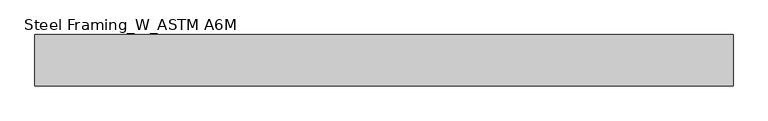
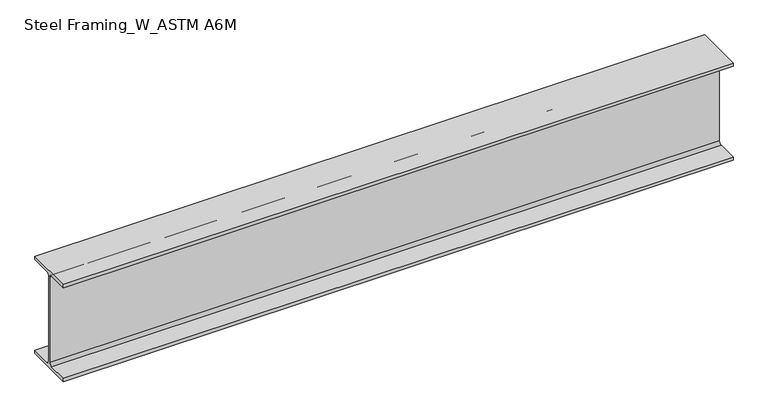
"""IFC4 building model written with IfcOpenShell, lengths in millimetres: beam geometry, Steel Framing_W_ASTM A6M : H_SB_AR_S02_W360x51_G3."""

import ifcopenshell
import ifcopenshell.guid

model = None  # the IFC model being written
_history = None  # IfcOwnerHistory: only IFC2X3 demands one
_inside = {}  # id of a spatial element -> (the spatial element, [elements in it])
_under = {}  # id of a project, library or spatial element -> (it, [spatial elements below it])
_declared = {}  # id of a project -> (the project, [libraries it declares])
_typed = {}  # id of a type object -> (the type object, [elements of that type])
_made_of = {}  # id of a material, layer set ... -> (it, [elements and type objects made of it])


def new_model(schema):
    """Start an empty IFC model of exactly this schema.

    Asked for "IFC4X3", IfcOpenShell would pick the latest addendum, in which some entities
    have other attributes; the version numbers below select the first issue.
    IFC2X3 requires an IfcOwnerHistory on every rooted entity: one is made here for all.
    """
    global model, _history
    if schema == "IFC4X3":
        model = ifcopenshell.file(schema_version=(4, 3, 0, 0))
    else:
        model = ifcopenshell.file(schema=schema)
    _inside.clear()
    _under.clear()
    _declared.clear()
    _typed.clear()
    _made_of.clear()
    _history = None
    if model.schema == "IFC2X3":
        org = make("IfcOrganization", Name="unknown")
        user = make(
            "IfcPersonAndOrganization",
            ThePerson=make("IfcPerson", FamilyName="unknown"),
            TheOrganization=org,
        )
        app = make(
            "IfcApplication",
            ApplicationDeveloper=org,
            Version="unknown",
            ApplicationFullName="unknown",
            ApplicationIdentifier="unknown",
        )
        _history = make(
            "IfcOwnerHistory",
            OwningUser=user,
            OwningApplication=app,
            ChangeAction="ADDED",
            CreationDate=0,
        )
    return model


def make(cls, **values):
    """One entity of the class cls with the attributes given. An attribute that is None is left unset."""
    return model.create_entity(
        cls, **{name: value for name, value in values.items() if value is not None}
    )


def rooted(cls, **values):
    """An entity with a GlobalId (a new one), such as an element, a storey or a relation."""
    return make(cls, GlobalId=ifcopenshell.guid.new(), OwnerHistory=_history, **values)


def si_unit(unit_type, name, prefix=None):
    """IfcSIUnit, for example si_unit("LENGTHUNIT", "METRE", prefix="MILLI")."""
    return make("IfcSIUnit", UnitType=unit_type, Prefix=prefix, Name=name)


def assignment(units):
    """IfcUnitAssignment: the units of a project."""
    return None if units is None else make("IfcUnitAssignment", Units=units)


def point(xyz):
    """IfcCartesianPoint."""
    return None if xyz is None else make("IfcCartesianPoint", Coordinates=xyz)


def direction(xyz):
    """IfcDirection."""
    return None if xyz is None else make("IfcDirection", DirectionRatios=xyz)


def frame(location, z_axis=None, x_axis=None):
    """IfcAxis2Placement3D, a coordinate frame: its origin and axes. An axis left out is left unset."""
    return make(
        "IfcAxis2Placement3D",
        Location=point(location),
        Axis=direction(z_axis),
        RefDirection=direction(x_axis),
    )


def frame_2d(location, x_axis=None):
    """IfcAxis2Placement2D, a coordinate frame in the plane: its origin and x axis."""
    return make(
        "IfcAxis2Placement2D", Location=point(location), RefDirection=direction(x_axis)
    )


def origin():
    """The frame at (0, 0, 0) with its axes left unset."""
    return frame((0.0, 0.0, 0.0))


def place(relative_to, where):
    """IfcLocalPlacement: puts the frame where relative to a parent placement (None: the world)."""
    return make(
        "IfcLocalPlacement", PlacementRelTo=relative_to, RelativePlacement=where
    )


def context(
    kind, dimensions, precision=None, world=None, true_north=None, identifier=None
):
    """IfcGeometricRepresentationContext, for example the 3D "Model" context."""
    return make(
        "IfcGeometricRepresentationContext",
        ContextIdentifier=identifier,
        ContextType=kind,
        CoordinateSpaceDimension=dimensions,
        Precision=precision,
        WorldCoordinateSystem=world,
        TrueNorth=true_north,
    )


def project(units=None, contexts=None):
    """IfcProject with its units and contexts."""
    return rooted(
        "IfcProject",
        Name="project",
        RepresentationContexts=contexts,
        UnitsInContext=assignment(units),
    )


def spatial(cls, under=None, at=None, **own):
    """A site, building, storey or space (cls), placed at a placement, below another one or the project."""
    s = rooted(cls, ObjectPlacement=at, **own)
    if under is not None:
        _under.setdefault(under.id(), (under, []))[1].append(s)
    return s


def polyline(points):
    """IfcPolyline through the points."""
    return make("IfcPolyline", Points=[point(p) for p in points])


def circle_curve(where, radius):
    """IfcCircle in the frame where."""
    return make("IfcCircle", Position=where, Radius=radius)


def trimmed(basis, trim1, trim2, sense, master):
    """IfcTrimmedCurve: the piece of a basis curve between two trims."""
    return make(
        "IfcTrimmedCurve",
        BasisCurve=basis,
        Trim1=trim1,
        Trim2=trim2,
        SenseAgreement=sense,
        MasterRepresentation=master,
    )


def segment(curve, same_sense, transition):
    """IfcCompositeCurveSegment."""
    return make(
        "IfcCompositeCurveSegment",
        Transition=transition,
        SameSense=same_sense,
        ParentCurve=curve,
    )


def composite_curve(segments, self_intersect=None):
    """IfcCompositeCurve: segments joined end to end."""
    return make("IfcCompositeCurve", Segments=segments, SelfIntersect=self_intersect)


def outline(outer, holes=None, kind="AREA"):
    """IfcArbitraryClosedProfileDef: a profile drawn as a closed curve; with holes, ...WithVoids."""
    if holes is None:
        return make("IfcArbitraryClosedProfileDef", ProfileType=kind, OuterCurve=outer)
    return make(
        "IfcArbitraryProfileDefWithVoids",
        ProfileType=kind,
        OuterCurve=outer,
        InnerCurves=holes,
    )


def extrude(swept, where, along, depth):
    """IfcExtrudedAreaSolid: the profile swept, set in the frame where, extruded along a direction by depth."""
    return make(
        "IfcExtrudedAreaSolid",
        SweptArea=swept,
        Position=where,
        ExtrudedDirection=direction(along),
        Depth=depth,
    )


def shape(context_of_items, identifier, shape_type, items):
    """IfcShapeRepresentation: the items that make up one representation, for example the "Body"."""
    return make(
        "IfcShapeRepresentation",
        ContextOfItems=context_of_items,
        RepresentationIdentifier=identifier,
        RepresentationType=shape_type,
        Items=items,
    )


def source(mapping_origin, context_of_items, identifier, shape_type, items):
    """IfcRepresentationMap: a shape defined once, which mapped items show again and again."""
    return make(
        "IfcRepresentationMap",
        MappingOrigin=mapping_origin,
        MappedRepresentation=shape(context_of_items, identifier, shape_type, items),
    )


def transform(
    local_origin,
    x_axis=None,
    y_axis=None,
    z_axis=None,
    scale=None,
    scale2=None,
    scale3=None,
    uniform=True,
):
    """IfcCartesianTransformationOperator3D, or its non-uniform kind. x_axis, y_axis, z_axis: its Axis1, 2, 3."""
    if uniform:
        return make(
            "IfcCartesianTransformationOperator3D",
            Axis1=direction(x_axis),
            Axis2=direction(y_axis),
            LocalOrigin=point(local_origin),
            Scale=scale,
            Axis3=direction(z_axis),
        )
    return make(
        "IfcCartesianTransformationOperator3DnonUniform",
        Axis1=direction(x_axis),
        Axis2=direction(y_axis),
        LocalOrigin=point(local_origin),
        Scale=scale,
        Axis3=direction(z_axis),
        Scale2=scale2,
        Scale3=scale3,
    )


def mapped(mapping_source, mapping_target):
    """IfcMappedItem: shows the shape of a source again, moved by a transform."""
    return make(
        "IfcMappedItem", MappingSource=mapping_source, MappingTarget=mapping_target
    )


def made_of(thing, what):
    """Note that an element or type object is made of a material, layer set ...; save() writes the relation."""
    if what is not None:
        _made_of.setdefault(what.id(), (what, []))[1].append(thing)
    return thing


def element(
    cls,
    number,
    at=None,
    inside=None,
    cuts=None,
    type_object=None,
    material=None,
    context=None,
    identifier="Body",
    shape_type=None,
    held_by="IfcProductDefinitionShape",
    body=None,
    shapes=None,
    **own,
):
    """One element of the class cls, such as IfcWall. Its Tag is "e" and its number.

    at: its placement. inside: the storey or other place that contains it. cuts: it is an
    opening in that element (IfcRelVoidsElement). A single representation is given by context,
    identifier, shape_type and body (its items); several are given by shapes. held_by: the class
    of the entity that holds the representations. save() writes the other relations.
    """
    e = rooted(cls, Tag="e%d" % number, ObjectPlacement=at, **own)
    if body is not None:
        shapes = [shape(context, identifier, shape_type, body)]
    if shapes is not None:
        e.Representation = make(held_by, Representations=shapes)
    if inside is not None:
        _inside.setdefault(inside.id(), (inside, []))[1].append(e)
    if cuts is not None:
        rooted(
            "IfcRelVoidsElement", RelatingBuildingElement=cuts, RelatedOpeningElement=e
        )
    if type_object is not None:
        _typed.setdefault(type_object.id(), (type_object, []))[1].append(e)
    return made_of(e, material)


def aggregate(whole, parts):
    """IfcRelAggregates: a whole, such as a stair, and the parts it consists of."""
    return rooted("IfcRelAggregates", RelatingObject=whole, RelatedObjects=parts)


def save(model, path):
    """Write the relations noted so far, then the file.

    IfcRelAggregates (storeys below a building ...), IfcRelContainedInSpatialStructure (elements
    in a storey), IfcRelDefinesByType, IfcRelAssociatesMaterial and IfcRelDeclares: one each for
    every whole, place, type object, material and project.
    """
    for whole, parts in _under.values():
        aggregate(whole, parts)
    for where, things in _inside.values():
        rooted(
            "IfcRelContainedInSpatialStructure",
            RelatedElements=things,
            RelatingStructure=where,
        )
    for kind, things in _typed.values():
        rooted("IfcRelDefinesByType", RelatedObjects=things, RelatingType=kind)
    for what, things in _made_of.values():
        rooted("IfcRelAssociatesMaterial", RelatedObjects=things, RelatingMaterial=what)
    for by, libraries in _declared.values():
        rooted("IfcRelDeclares", RelatingContext=by, RelatedDefinitions=libraries)
    model.write(path)


def steel_framing_w_astm_a6m_44bd27a9(model_context):
    return source(origin(), model_context, "Body", "SweptSolid", [
        extrude(outline(composite_curve([segment(polyline([(85.5, -166.4), (85.5, -178.0), (-85.5, -178.0), (-85.5, -166.4), (-13.72, -166.4)]), True, "CONTINUOUS"), segment(trimmed(circle_curve(frame_2d((-13.72, -156.3)), 10.1), [point((-13.72, -166.4))], [point((-3.62, -156.3))], True, "CARTESIAN"), True, "CONTINUOUS"), segment(polyline([(-3.62, -156.3), (-3.62, 156.3)]), True, "CONTINUOUS"), segment(trimmed(circle_curve(frame_2d((-13.72, 156.3)), 10.1), [point((-3.62, 156.3))], [point((-13.72, 166.4))], True, "CARTESIAN"), True, "CONTINUOUS"), segment(polyline([(-13.72, 166.4), (-85.5, 166.4), (-85.5, 178.0), (85.5, 178.0), (85.5, 166.4), (13.72, 166.4)]), True, "CONTINUOUS"), segment(trimmed(circle_curve(frame_2d((13.72, 156.3)), 10.1), [point((13.72, 166.4))], [point((3.62, 156.3))], True, "CARTESIAN"), True, "CONTINUOUS"), segment(polyline([(3.62, 156.3), (3.62, -156.3)]), True, "CONTINUOUS"), segment(trimmed(circle_curve(frame_2d((13.72, -156.3)), 10.1), [point((3.62, -156.3))], [point((13.72, -166.4))], True, "CARTESIAN"), True, "CONTINUOUS"), segment(polyline([(13.72, -166.4), (85.5, -166.4)]), True, "CONTINUOUS")], self_intersect=False)), frame((-1003.8, 0.0, 0.0), z_axis=(1.0, 0.0, 0.0), x_axis=(0.0, 1.0, 0.0)), (0.0, 0.0, 1.0), 2320.8),
    ])


if __name__ == "__main__":
    model = new_model("IFC4")
    model_context = context("Model", 3, world=origin())
    ifc_project = project(units=[si_unit("LENGTHUNIT", "METRE", prefix="MILLI")], contexts=[model_context])
    site = spatial("IfcSite", under=ifc_project)
    building = spatial("IfcBuilding", under=site)
    placement = place(None, origin())
    steel_framing_w_astm_a6m_shape = steel_framing_w_astm_a6m_44bd27a9(model_context)
    element("IfcBeam", 1, ObjectType="Steel Framing_W_ASTM A6M : H_SB_AR_S02_W360x51_G3", at=placement, inside=building, context=model_context, shape_type="MappedRepresentation", body=[
        mapped(steel_framing_w_astm_a6m_shape, transform((0.0, 0.0, 0.0), x_axis=(1.0, 0.0, 0.0), y_axis=(0.0, 1.0, 0.0), z_axis=(0.0, 0.0, 1.0))),
    ])
    save(model, "model.ifc")

# Revit data of these elements
# Type "Steel Framing_W_ASTM A6M : H_SB_AR_S02_W360x51_G3"
#   Type Mark = "G3"
#   Section Name Key = "W14x34"
#   Width = 17.1 cm
#   Web Thickness = 0.724 cm
#   Web Fillet = 1.01 cm
#   Warping Constant = 287000.0 cm⁶
#   Torsional Moment of Inertia = 23.70 cm⁴
#   Section Area = 64.5 cm²
#   Plastic Modulus weak axis = 174.0 cm³
#   Plastic Modulus strong axis = 895.0 cm³
#   Perimeter = 1.36 m²/m
#   Nominal Weight = 51.00 kgf/m
#   Moment of Inertia weak axis = 970.00 cm⁴
#   Moment of Inertia strong axis = 14200.00 cm⁴
#   Height = 35.6 cm
#   Flange Thickness = 1.16 cm
#   Elastic Modulus weak axis = 113.0 cm³
#   Elastic Modulus strong axis = 796.0 cm³
#   Centroid Vertical = 17.8 cm
#   Centroid Horizontal = 8.55 cm
#   Length [instance default] = 1500 mm
#   Structural Material [instance default] = Steel, 45-345
#   Bolt Spacing = 0
#   Assembly Code = ""
# Element 1 (IfcBeam, "Steel Framing_W_ASTM A6M : H_SB_AR_S02_W360x51_G3")
#   Materials on its faces: "Steel, 45-345"
# Materials
#   "Steel, 45-345": class "Metal", colour RGB 189 187 185, transparency 0, Description = "Steel 345 MPa", Cost = 0
